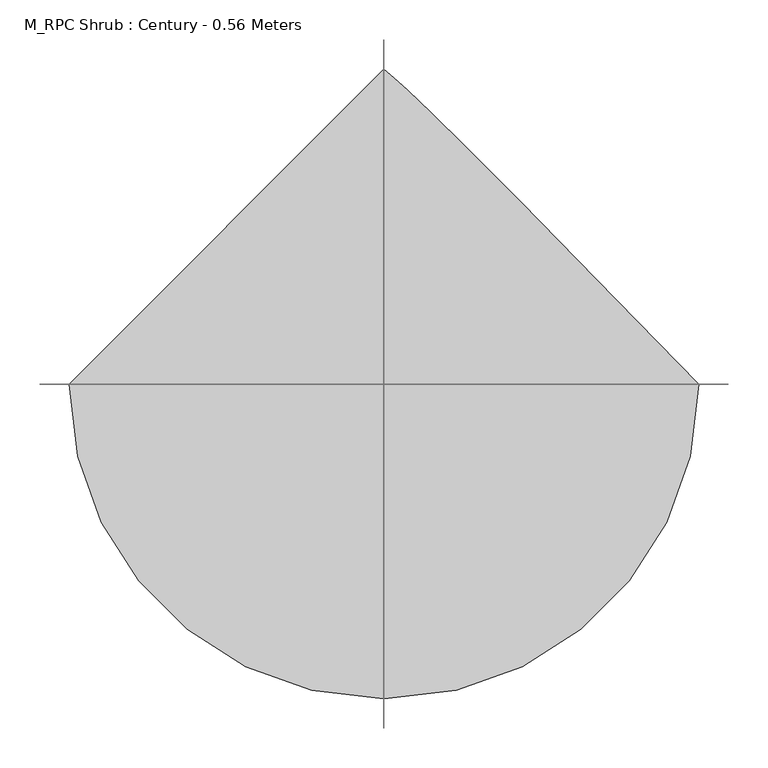
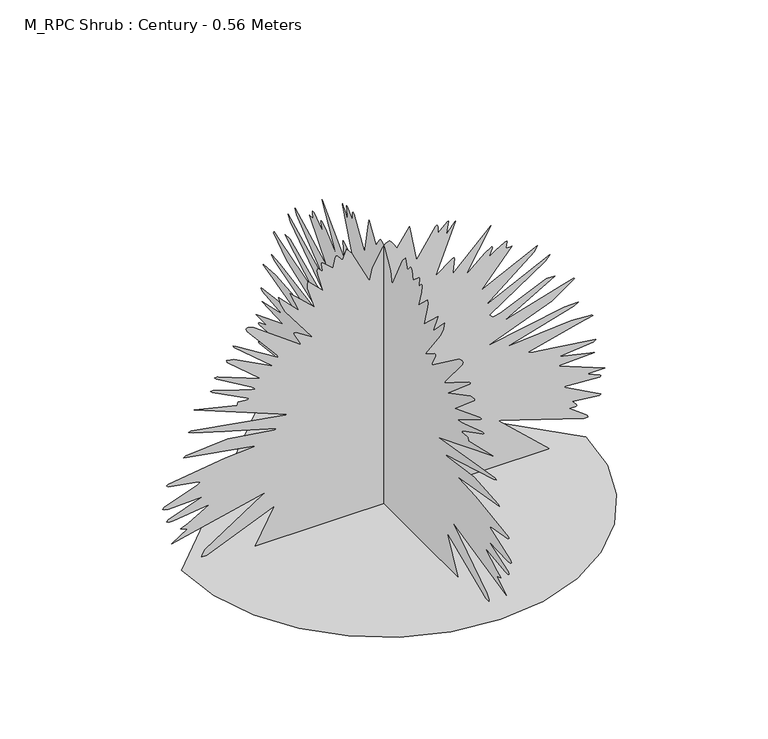
"""IFC4 building model written with IfcOpenShell, lengths in millimetres: geographic element geometry, M_RPC Shrub : Century - 0.56 Meters."""

from ifc_helpers import new_model, si_unit, origin, place, context, project, spatial, triangles, source, transform, mapped, element, save


def m_rpc_shrub_century_0_56_meters_67d26a43(model_context):
    return source(origin(), model_context, "Body", "Tessellation", [
        triangles([(-398.1646863, 0.0, 4.64e-05), (-387.6392386, -91.2330759, 4.64e-05), (-357.6589102, -175.0158616, 4.64e-05), (-310.62915, -248.9482674, 4.64e-05), (-248.9482674, -310.62915, 4.64e-05), (-175.0158616, -357.6589102, 4.64e-05), (-91.2330759, -387.6392386, 4.64e-05), (1.74e-05, -398.1646863, 4.64e-05), (91.2330759, -387.6392386, 4.64e-05), (175.0158616, -357.6589102, 4.64e-05), (248.9482674, -310.62915, 4.64e-05), (310.62915, -248.9482674, 4.64e-05), (357.6589102, -175.0158616, 4.64e-05), (387.6392386, -91.2330759, 4.64e-05), (398.1646863, 3.48e-05, 4.64e-05), (268.7691869, 132.7272546, 4.64e-05), (172.8430654, 230.4484337, 4.64e-05), (104.8064389, 298.9964298, 4.64e-05), (59.0817226, 344.2087501, 4.64e-05), (30.0910616, 371.9185412, 4.64e-05), (12.2565295, 387.9599676, 4.64e-05), (-5.22e-05, 398.1646863, 4.64e-05), (5.49e-05, 64.8497162, 484.8984183), (5.49e-05, 101.536553, 542.1176365), (5.49e-05, 104.7998259, 543.9987353), (5.48e-05, 106.0554996, 542.5580166), (5.48e-05, 106.6816787, 540.4605792), (5.49e-05, 106.3998917, 526.3994825), (5.49e-05, 126.0240573, 543.3318429), (5.49e-05, 127.1998031, 543.9987353), (5.49e-05, 124.5247847, 525.7834954), (5.49e-05, 123.9199888, 519.3689524), (5.49e-05, 123.9999166, 518.3991351), (5.49e-05, 126.4310728, 521.7234962), (5.49e-05, 129.404674, 525.5416497), (5.49e-05, 132.6114368, 529.4820342), (5.49e-05, 135.7433586, 533.1856599), (5.49e-05, 138.4909199, 536.2834723), (5.49e-05, 140.5461178, 538.4089239), (5.49e-05, 141.5999325, 539.2005544), (5.49e-05, 101.5999394, 438.4006751), (5.49e-05, 135.4317952, 463.1119211), (5.49e-05, 138.3997917, 464.0002753), (5.47e-05, 139.1298253, 461.7042672), (5.51e-05, 136.2157953, 434.8777433), (5.49e-05, 136.7999711, 431.9988493), (5.49e-05, 211.4496842, 505.8500464), (5.49e-05, 160.799778, 419.2003209), (5.45e-05, 199.0650477, 452.2453606), (5.47e-05, 210.839547, 460.3373812), (5.49e-05, 213.5998255, 460.8006523), (5.49e-05, 214.2417921, 458.8177428), (5.49e-05, 213.7067412, 456.0762677), (5.5e-05, 208.6102318, 443.5832076), (5.49e-05, 208.7998641, 441.6002981), (5.47e-05, 220.3880376, 450.0359387), (5.47e-05, 238.7186048, 461.4981025), (5.49e-05, 242.3998299, 462.3991739), (5.49e-05, 242.9542292, 460.7548339), (5.49e-05, 240.6740268, 448.6562991), (5.49e-05, 240.7997641, 447.9995441), (5.49e-05, 241.2714286, 448.0708334), (5.49e-05, 242.5398286, 447.9257478), (5.49e-05, 244.3852829, 447.6737283), (5.49e-05, 246.5886367, 447.426832), (5.49e-05, 248.9301908, 447.2919202), (5.49e-05, 251.1902999, 447.3810136), (5.49e-05, 253.1497915, 447.7984663), (5.49e-05, 192.7999141, 377.5999895), (5.49e-05, 303.1989713, 431.9988493), (5.49e-05, 297.1993375, 421.8501228), (5.49e-05, 199.199687, 342.3989405), (5.49e-05, 327.2000499, 404.8006911), (5.49e-05, 318.9502264, 393.7992551), (5.49e-05, 208.7998641, 319.9989633), (5.49e-05, 215.1998913, 313.5996809), (5.49e-05, 230.1625681, 316.3946048), (5.49e-05, 320.6811527, 356.7196507), (5.49e-05, 337.1502056, 356.6483614), (5.49e-05, 238.1998319, 298.4491704), (5.49e-05, 354.9760071, 333.6273102), (5.49e-05, 375.1996273, 339.1993175), (5.49e-05, 375.7138038, 337.4455001), (5.49e-05, 331.4993151, 306.2993271), (5.49e-05, 203.9999027, 257.5997561), (5.49e-05, 355.6938412, 284.8055446), (5.49e-05, 383.1999747, 286.3989974), (5.49e-05, 374.9501876, 280.4986309), (5.49e-05, 243.9996596, 241.5998061), (5.49e-05, 369.6149028, 252.730304), (5.48e-05, 410.4057632, 249.1238926), (5.49e-05, 411.9992343, 247.9998333), (5.49e-05, 387.0894539, 241.9686426), (5.49e-05, 285.2993553, 215.7497124), (5.49e-05, 290.8815363, 213.1882227), (5.49e-05, 337.9749372, 207.3566019), (5.49e-05, 416.616685, 196.3696635), (5.49e-05, 418.3985167, 195.1997676), (5.52e-05, 413.4781411, 191.71199), (5.49e-05, 346.4004041, 185.5998631), (5.49e-05, 415.1988573, 169.5999131), (5.49e-05, 343.2007447, 166.3997632), (5.49e-05, 436.0003129, 129.599911), (5.49e-05, 400.7992275, 129.599911), (5.49e-05, 426.360676, 118.4839198), (5.49e-05, 427.9999291, 116.7998474), (5.51e-05, 425.8286591, 115.4250494), (5.56e-05, 353.1509368, 119.8681376), (5.49e-05, 427.9999291, 78.3999202), (5.49e-05, 425.4595682, 76.8158872), (5.49e-05, 372.0000043, 83.1998816), (5.49e-05, 379.473458, 73.9621824), (5.49e-05, 380.2828926, 71.8871274), (5.49e-05, 380.0003517, 70.3998226), (5.5e-05, 378.39162, 69.8721477), (5.49e-05, 365.6007219, 70.3998226), (5.51e-05, 397.7981389, 47.0083907), (5.51e-05, 401.3999539, 43.1362478), (5.49e-05, 402.4003289, 39.9999976), (5.52e-05, 394.3261488, 39.8897799), (5.49e-05, 224.7995597, 94.3998702), (5.49e-05, 327.2000499, 0.0), (5.26e-05, -253.5998185, 0.2497534), (5.49e-05, -215.1998913, 70.3998226), (5.53e-05, -349.5058468, 14.9203965), (5.49e-05, -359.1989325, 14.3999784), (5.49e-05, -358.4582073, 18.4088623), (5.49e-05, -352.929475, 27.5733556), (5.49e-05, -237.8852254, 102.3824044), (5.49e-05, -229.5997755, 105.5998588), (5.49e-05, -418.3985167, 62.3999748), (5.49e-05, -386.3996341, 83.1998816), (5.49e-05, -400.0025102, 87.4296561), (5.49e-05, -400.7992275, 87.999843), (5.49e-05, -386.0559777, 93.9304857), (5.49e-05, -343.2007447, 118.3999223), (5.53e-05, -414.9570479, 109.1403313), (5.52e-05, -423.9373864, 109.6170918), (5.49e-05, -427.9999291, 111.999886), (5.47e-05, -424.9504786, 115.4097796), (5.49e-05, -357.6003745, 139.1998246), (5.52e-05, -424.695952, 136.9435397), (5.52e-05, -432.7879363, 138.2035373), (5.49e-05, -436.0003129, 140.7998996), (5.49e-05, -432.057385, 144.8611706), (5.51e-05, -366.8785509, 167.9405303), (5.49e-05, -362.3985555, 171.1997246), (5.48e-05, -365.5549035, 173.2315046), (5.52e-05, -424.548323, 183.6813392), (5.49e-05, -427.9999291, 187.1996746), (5.5e-05, -424.9912102, 188.5632723), (5.5e-05, -312.2404252, 204.2493606), (5.5e-05, -256.8437521, 207.9244815), (5.49e-05, -253.5998185, 209.5996518), (5.49e-05, -394.3999815, 233.5996948), (5.47e-05, -390.436706, 236.3123926), (5.49e-05, -308.2873235, 242.4260456), (5.52e-05, -215.1914979, 228.4782414), (5.49e-05, -210.3996938, 230.3998175), (5.5e-05, -317.0436931, 261.3695659), (5.51e-05, -375.8232811, 278.6964516), (5.49e-05, -384.7985327, 283.1993563), (5.48e-05, -379.7305281, 284.1615432), (5.49e-05, -186.3998869, 251.1997107), (5.49e-05, -373.5985259, 326.4007891), (5.49e-05, -288.7993597, 305.5993335), (5.49e-05, -287.2008017, 311.9986158), (5.5e-05, -269.6142843, 310.6546208), (5.5e-05, -267.4048262, 311.0720736), (5.49e-05, -266.3993824, 311.9986158), (5.52e-05, -270.0673635, 315.259318), (5.51e-05, -338.1327765, 350.2134707), (5.49e-05, -341.5996797, 353.5989109), (5.49e-05, -336.2949526, 353.3087397), (5.54e-05, -272.2895571, 332.4284008), (5.53e-05, -259.5164814, 328.6509424), (5.49e-05, -253.5998185, 327.9993107), (5.48e-05, -256.7444849, 331.695306), (5.51e-05, -330.0891177, 375.2072577), (5.49e-05, -333.5992959, 379.1985475), (5.48e-05, -328.2309463, 379.1425552), (5.49e-05, -242.3998299, 345.5985635), (5.51e-05, -308.8677023, 402.8279554), (5.49e-05, -309.6007971, 406.3992491), (5.49e-05, -295.3818975, 403.9785029), (5.49e-05, -218.3997869, 363.2003597), (5.5e-05, -295.1171608, 428.5930252), (5.49e-05, -296.7997071, 431.9988493), (5.43e-05, -290.6473573, 429.7792173), (5.43e-05, -242.0870038, 399.1116125), (5.49e-05, -207.1997983, 377.5999895), (5.5e-05, -209.9585506, 383.227989), (5.51e-05, -269.0008225, 453.4340961), (5.49e-05, -271.2001069, 459.1995509), (5.48e-05, -269.5073686, 460.136267), (5.48e-05, -267.1197418, 460.2660919), (5.49e-05, -256.5637546, 456.7737179), (5.49e-05, -163.9999097, 388.7999963), (5.51e-05, -163.8922309, 391.6330719), (5.51e-05, -177.0634292, 415.4890649), (5.49e-05, -176.7997098, 417.5992195), (5.46e-05, -172.6549592, 417.5126696), (5.49e-05, -139.9998666, 396.8003437), (5.49e-05, -194.1836233, 468.5159154), (5.49e-05, -203.5692241, 486.9984355), (5.49e-05, -207.1997983, 502.3984039), (5.49e-05, -167.1998052, 460.8006523), (5.49e-05, -184.799821, 502.3984039), (5.49e-05, -136.7999711, 457.5984495), (5.49e-05, -150.0974153, 501.1027708), (5.49e-05, -150.4718564, 508.5049716), (5.49e-05, -149.5997803, 515.1995121), (5.49e-05, -119.1999553, 486.4002525), (5.44e-05, -128.5677247, 518.5645683), (5.46e-05, -131.0228165, 531.0958529), (5.49e-05, -130.3999439, 534.39983), (5.48e-05, -129.2058761, 534.7740077), (5.48e-05, -127.886816, 534.1198325), (5.5e-05, -121.9235899, 527.8402013), (5.5e-05, -120.4008994, 527.0129262), (5.5e-05, -120.2359567, 529.3420355), (5.49e-05, -122.5647935, 541.6518219), (5.49e-05, -122.3998417, 543.9987353), (5.47e-05, -119.8953707, 543.5074499), (5.49e-05, -102.2846633, 527.55003), (5.49e-05, -99.9998645, 526.3994825), (5.47e-05, -96.0065581, 544.5052814), (5.48e-05, -94.9280538, 547.1169316), (5.49e-05, -93.5998373, 548.7994597), (5.48e-05, -91.4494416, 548.2191173), (5.49e-05, -80.8000281, 535.9983879), (5.49e-05, -73.8677477, 555.4583556), (5.49e-05, -73.4500361, 555.949641), (5.49e-05, -63.3254997, 544.6173022), (5.49e-05, -27.9999715, 473.5991807), (5.45e-05, -22.4632319, 499.4533439), (5.39e-05, -2.4030595, 534.758747), (5.42e-05, 4.5359445, 541.494019), (5.49e-05, 10.3999784, 543.9987353), (5.49e-05, 12.3719147, 542.8354706), (5.49e-05, 15.0237162, 539.8598528), (5.49e-05, 18.0101936, 535.7973101), (5.49e-05, 20.9862349, 531.3758503), (5.49e-05, 23.6065737, 527.315851), (5.49e-05, 25.5263012, 524.350407), (5.49e-05, 26.3999011, 523.1998595), (5.49e-05, 50.3999487, 559.9994665), (64.8497162, 5.25e-05, 484.8984183), (101.536553, 4.91e-05, 542.1176365), (104.7998259, 4.9e-05, 543.9987353), (106.0554996, 4.92e-05, 542.5580166), (106.6816787, 4.93e-05, 540.4605792), (106.3998917, 5e-05, 526.3994825), (126.0240573, 4.9e-05, 543.3318429), (127.1998031, 4.9e-05, 543.9987353), (124.5247847, 5e-05, 525.7834954), (123.9199888, 5.04e-05, 519.3689524), (123.9999166, 5.05e-05, 518.3991351), (126.4310728, 5.03e-05, 521.7234962), (129.404674, 5.01e-05, 525.5416497), (132.6114368, 4.98e-05, 529.4820342), (135.7433586, 4.96e-05, 533.1856599), (138.4909199, 4.94e-05, 536.2834723), (140.5461178, 4.93e-05, 538.4089239), (141.5999325, 4.92e-05, 539.2005544), (101.5999394, 5.52e-05, 438.4006751), (135.4317952, 5.38e-05, 463.1119211), (138.3997917, 5.37e-05, 464.0002753), (139.1298253, 5.41e-05, 461.7042672), (136.2157953, 5.53e-05, 434.8777433), (136.7999711, 5.56e-05, 431.9988493), (211.4496842, 5.12e-05, 505.8500464), (160.799778, 5.64e-05, 419.2003209), (199.0650477, 5.48e-05, 452.2453606), (210.839547, 5.42e-05, 460.3373812), (213.5998255, 5.39e-05, 460.8006523), (214.2417921, 5.41e-05, 458.8177428), (213.7067412, 5.43e-05, 456.0762677), (208.6102318, 5.49e-05, 443.5832076), (208.7998641, 5.51e-05, 441.6002981), (220.3880376, 5.48e-05, 450.0359387), (238.7186048, 5.41e-05, 461.4981025), (242.3998299, 5.38e-05, 462.3991739), (242.9542292, 5.4e-05, 460.7548339), (240.6740268, 5.46e-05, 448.6562991), (240.7997641, 5.47e-05, 447.9995441), (241.2714286, 5.47e-05, 448.0708334), (242.5398286, 5.47e-05, 447.9257478), (244.3852829, 5.47e-05, 447.6737283), (246.5886367, 5.47e-05, 447.426832), (248.9301908, 5.47e-05, 447.2919202), (251.1902999, 5.47e-05, 447.3810136), (253.1497915, 5.47e-05, 447.7984663), (192.7999141, 5.89e-05, 377.5999895), (303.1989713, 5.56e-05, 431.9988493), (297.1993375, 5.62e-05, 421.8501228), (199.199687, 6.1e-05, 342.3989405), (327.2000499, 5.73e-05, 404.8006911), (318.9502264, 5.79e-05, 393.7992551), (208.7998641, 6.23e-05, 319.9989633), (215.1998913, 6.27e-05, 313.5996809), (230.1625681, 6.25e-05, 316.3946048), (320.6811527, 6.01e-05, 356.7196507), (337.1502056, 6.01e-05, 356.6483614), (238.1998319, 6.36e-05, 298.4491704), (354.9760071, 6.15e-05, 333.6273102), (375.1996273, 6.12e-05, 339.1993175), (375.7138038, 6.13e-05, 337.4455001), (331.4993151, 6.31e-05, 306.2993271), (203.9999027, 6.6e-05, 257.5997561), (355.6938412, 6.44e-05, 284.8055446), (383.1999747, 6.43e-05, 286.3989974), (374.9501876, 6.47e-05, 280.4986309), (243.9996596, 6.7e-05, 241.5998061), (369.6149028, 6.63e-05, 252.730304), (410.4057632, 6.66e-05, 249.1238926), (411.9992343, 6.66e-05, 247.9998333), (387.0894539, 6.7e-05, 241.9686426), (285.2993553, 6.85e-05, 215.7497124), (290.8815363, 6.87e-05, 213.1882227), (337.9749372, 6.9e-05, 207.3566019), (416.616685, 6.97e-05, 196.3696635), (418.3985167, 6.97e-05, 195.1997676), (413.4781411, 6.96e-05, 191.71199), (346.4004041, 7.03e-05, 185.5998631), (415.1988573, 7.13e-05, 169.5999131), (343.2007447, 7.15e-05, 166.3997632), (436.0003129, 7.37e-05, 129.599911), (400.7992275, 7.37e-05, 129.599911), (426.360676, 7.43e-05, 118.4839198), (427.9999291, 7.44e-05, 116.7998474), (425.8286591, 7.43e-05, 115.4250494), (353.1509368, 7.36e-05, 119.8681376), (427.9999291, 7.67e-05, 78.3999202), (425.4595682, 7.68e-05, 76.8158872), (372.0000043, 7.64e-05, 83.1998816), (379.473458, 7.7e-05, 73.9621824), (380.2828926, 7.71e-05, 71.8871274), (380.0003517, 7.72e-05, 70.3998226), (378.39162, 7.71e-05, 69.8721477), (365.6007219, 7.72e-05, 70.3998226), (397.7981389, 7.84e-05, 47.0083907), (401.3999539, 7.87e-05, 43.1362478), (402.4003289, 7.9e-05, 39.9999976), (394.3261488, 7.87e-05, 39.8897799), (224.7995597, 7.58e-05, 94.3998702), (327.2000499, 8.14e-05, 1.09e-05), (-253.5998185, 8.37e-05, 0.2497643), (-215.1998913, 7.72e-05, 70.3998226), (-349.5058468, 8.01e-05, 14.9204215), (-359.1989325, 8.05e-05, 14.4000045), (-358.4582073, 8.03e-05, 18.4088623), (-352.929475, 7.97e-05, 27.5733556), (-237.8852254, 7.53e-05, 102.3824044), (-229.5997755, 7.51e-05, 105.5998588), (-418.3985167, 7.77e-05, 62.3999748), (-386.3996341, 7.64e-05, 83.1998816), (-400.0025102, 7.62e-05, 87.4296561), (-400.7992275, 7.61e-05, 87.999843), (-386.0559777, 7.58e-05, 93.9304857), (-343.2007447, 7.43e-05, 118.3999223), (-414.9570479, 7.46e-05, 109.1403313), (-423.9373864, 7.46e-05, 109.6170918), (-427.9999291, 7.47e-05, 111.999886), (-424.9504786, 7.47e-05, 115.4097796), (-357.6003745, 7.31e-05, 139.1998246), (-424.695952, 7.29e-05, 136.9435397), (-432.7879363, 7.29e-05, 138.2035373), (-436.0003129, 7.3e-05, 140.7998996), (-432.057385, 7.28e-05, 144.8611706), (-366.8785509, 7.12e-05, 167.9405303), (-362.3985555, 7.12e-05, 171.1997246), (-365.5549035, 7.11e-05, 173.2315046), (-424.548323, 7.02e-05, 183.6813392), (-427.9999291, 7.02e-05, 187.1996746), (-424.9912102, 7.01e-05, 188.5632723), (-312.2404252, 6.92e-05, 204.2493606), (-256.8437521, 6.89e-05, 207.9244815), (-253.5998185, 6.89e-05, 209.5996518), (-394.3999815, 6.75e-05, 233.5996948), (-390.436706, 6.75e-05, 236.3123926), (-308.2873235, 6.7e-05, 242.4260456), (-215.1914979, 6.75e-05, 228.4782414), (-210.3996938, 6.76e-05, 230.3998175), (-317.0436931, 6.57e-05, 261.3695659), (-375.8232811, 6.46e-05, 278.6964516), (-384.7985327, 6.45e-05, 283.1993563), (-379.7305281, 6.46e-05, 284.1615432), (-186.3998869, 6.64e-05, 251.1997107), (-373.5985259, 6.19e-05, 326.4007891), (-288.7993597, 6.32e-05, 305.5993335), (-287.2008017, 6.28e-05, 311.9986158), (-269.6142843, 6.28e-05, 310.6546208), (-267.4048262, 6.28e-05, 311.0720736), (-266.3993824, 6.28e-05, 311.9986158), (-270.0673635, 6.23e-05, 315.259318), (-338.1327765, 6.04e-05, 350.2134707), (-341.5996797, 6.03e-05, 353.5989109), (-336.2949526, 6.04e-05, 353.3087397), (-272.2895571, 6.11e-05, 332.4284008), (-259.5164814, 6.14e-05, 328.6509424), (-253.5998185, 6.18e-05, 327.9993107), (-256.7444849, 6.17e-05, 331.695306), (-330.0891177, 5.89e-05, 375.2072577), (-333.5992959, 5.88e-05, 379.1985475), (-328.2309463, 5.89e-05, 379.1425552), (-242.3998299, 6.08e-05, 345.5985635), (-308.8677023, 5.72e-05, 402.8279554), (-309.6007971, 5.72e-05, 406.3992491), (-295.3818975, 5.73e-05, 403.9785029), (-218.3997869, 5.97e-05, 363.2003597), (-295.1171608, 5.58e-05, 428.5930252), (-296.7997071, 5.56e-05, 431.9988493), (-290.6473573, 5.64e-05, 429.7792173), (-242.0870038, 5.82e-05, 399.1116125), (-207.1997983, 5.89e-05, 377.5999895), (-209.9585506, 5.85e-05, 383.227989), (-269.0008225, 5.42e-05, 453.4340961), (-271.2001069, 5.4e-05, 459.1995509), (-269.5073686, 5.41e-05, 460.136267), (-267.1197418, 5.41e-05, 460.2660919), (-256.5637546, 5.42e-05, 456.7737179), (-163.9999097, 5.82e-05, 388.7999963), (-163.8922309, 5.78e-05, 391.6330719), (-177.0634292, 5.65e-05, 415.4890649), (-176.7997098, 5.65e-05, 417.5992195), (-172.6549592, 5.68e-05, 417.5126696), (-139.9998666, 5.77e-05, 396.8003437), (-194.1836233, 5.35e-05, 468.5159154), (-203.5692241, 5.24e-05, 486.9984355), (-207.1997983, 5.14e-05, 502.3984039), (-167.1998052, 5.39e-05, 460.8006523), (-184.799821, 5.14e-05, 502.3984039), (-136.7999711, 5.41e-05, 457.5984495), (-150.0974153, 5.15e-05, 501.1027708), (-150.4718564, 5.11e-05, 508.5049716), (-149.5997803, 5.07e-05, 515.1995121), (-119.1999553, 5.24e-05, 486.4002525), (-128.5677247, 5.1e-05, 518.5645683), (-131.0228165, 5.01e-05, 531.0958529), (-130.3999439, 4.95e-05, 534.39983), (-129.2058761, 4.96e-05, 534.7740077), (-127.886816, 4.96e-05, 534.1198325), (-121.9235899, 4.98e-05, 527.8402013), (-120.4008994, 4.99e-05, 527.0129262), (-120.2359567, 4.97e-05, 529.3420355), (-122.5647935, 4.91e-05, 541.6518219), (-122.3998417, 4.9e-05, 543.9987353), (-119.8953707, 4.92e-05, 543.5074499), (-102.2846633, 5e-05, 527.55003), (-99.9998645, 5e-05, 526.3994825), (-96.0065581, 4.91e-05, 544.5052814), (-94.9280538, 4.89e-05, 547.1169316), (-93.5998373, 4.87e-05, 548.7994597), (-91.4494416, 4.88e-05, 548.2191173), (-80.8000281, 4.94e-05, 535.9983879), (-73.8677477, 4.83e-05, 555.4583556), (-73.4500361, 4.82e-05, 555.949641), (-63.3254997, 4.89e-05, 544.6173022), (-27.9999715, 5.32e-05, 473.5991807), (-22.4632319, 5.2e-05, 499.4533439), (-2.4030595, 5.05e-05, 534.758747), (4.5359445, 4.98e-05, 541.494019), (10.3999784, 4.9e-05, 543.9987353), (12.3719147, 4.9e-05, 542.8354706), (15.0237162, 4.92e-05, 539.8598528), (18.0101936, 4.94e-05, 535.7973101), (20.9862349, 4.97e-05, 531.3758503), (23.6065737, 4.99e-05, 527.315851), (25.5263012, 5.01e-05, 524.350407), (26.3999011, 5.02e-05, 523.1998595), (50.3999487, 4.8e-05, 559.9994665)], [[21, 22, 1], [20, 21, 1], [19, 20, 1], [18, 19, 1], [17, 18, 1], [17, 1, 2], [17, 2, 3], [17, 3, 4], [16, 17, 4], [16, 4, 5], [16, 5, 6], [16, 6, 7], [16, 7, 8], [16, 8, 9], [16, 9, 10], [16, 10, 11], [16, 11, 12], [15, 16, 12], [14, 15, 12], [13, 14, 12], [164, 165, 166], [46, 47, 48], [100, 101, 102], [130, 131, 132], [102, 103, 104], [207, 208, 209], [72, 73, 74], [72, 74, 75], [205, 206, 207], [204, 205, 207], [78, 79, 80], [39, 40, 41], [38, 39, 41], [37, 38, 41], [36, 37, 41], [35, 36, 41], [34, 35, 41], [33, 34, 41], [86, 87, 88], [86, 88, 89], [69, 70, 71], [69, 71, 72], [67, 68, 69], [161, 162, 163], [172, 173, 174], [121, 122, 123], [187, 188, 189], [246, 247, 23], [154, 155, 156], [154, 156, 157], [77, 78, 80], [66, 67, 69], [179, 180, 181], [91, 92, 93], [90, 91, 93], [121, 123, 124], [29, 30, 31], [133, 134, 135], [132, 133, 135], [211, 212, 213], [210, 211, 213], [65, 66, 69], [85, 86, 89], [64, 65, 69], [187, 189, 190], [186, 187, 190], [108, 109, 110], [108, 110, 111], [63, 64, 69], [62, 63, 69], [61, 62, 69], [97, 98, 99], [183, 184, 185], [149, 150, 151], [118, 119, 120], [117, 118, 120], [125, 126, 127], [105, 106, 107], [138, 139, 140], [160, 161, 163], [160, 163, 164], [159, 160, 164], [232, 233, 234], [231, 232, 234], [222, 223, 224], [186, 190, 191], [143, 144, 145], [96, 97, 99], [172, 174, 175], [171, 172, 175], [171, 175, 176], [81, 82, 83], [81, 83, 84], [42, 43, 44], [96, 99, 100], [182, 183, 185], [142, 143, 145], [141, 142, 145], [170, 171, 176], [203, 204, 207], [203, 207, 209], [141, 145, 146], [57, 58, 59], [89, 90, 93], [89, 93, 94], [81, 84, 85], [80, 81, 85], [200, 201, 202], [148, 149, 151], [148, 151, 152], [178, 179, 181], [178, 181, 182], [177, 178, 182], [193, 194, 195], [193, 195, 196], [166, 167, 168], [164, 166, 168], [164, 168, 169], [164, 169, 170], [50, 51, 52], [116, 117, 120], [24, 25, 26], [24, 26, 27], [137, 138, 140], [136, 137, 140], [136, 140, 141], [50, 52, 53], [49, 50, 53], [49, 53, 54], [49, 54, 55], [76, 77, 80], [76, 80, 85], [125, 127, 128], [124, 125, 128], [124, 128, 129], [124, 129, 130], [199, 200, 202], [182, 185, 186], [147, 148, 152], [164, 170, 176], [164, 176, 177], [104, 105, 107], [104, 107, 108], [102, 104, 108], [193, 196, 197], [192, 193, 197], [192, 197, 198], [191, 192, 198], [164, 177, 182], [164, 182, 186], [141, 146, 147], [130, 132, 135], [130, 135, 136], [121, 124, 130], [221, 222, 224], [28, 29, 31], [28, 31, 32], [41, 42, 44], [41, 44, 45], [23, 24, 27], [23, 27, 28], [209, 210, 213], [199, 202, 203], [198, 199, 203], [221, 224, 225], [220, 221, 225], [154, 157, 158], [228, 229, 230], [56, 57, 59], [56, 59, 60], [116, 120, 121], [28, 32, 33], [28, 33, 41], [23, 28, 41], [215, 216, 217], [215, 217, 218], [214, 215, 218], [214, 218, 219], [214, 219, 220], [113, 114, 115], [112, 113, 115], [111, 112, 115], [41, 45, 46], [111, 115, 116], [214, 220, 225], [214, 225, 226], [96, 100, 102], [56, 60, 61], [56, 61, 69], [55, 56, 69], [49, 55, 69], [48, 49, 69], [111, 116, 121], [108, 111, 121], [102, 108, 121], [96, 102, 121], [95, 96, 121], [94, 95, 121], [89, 94, 121], [89, 121, 130], [85, 89, 130], [76, 85, 130], [75, 76, 130], [72, 75, 130], [69, 72, 130], [48, 69, 130], [46, 48, 130], [41, 46, 130], [23, 41, 130], [246, 23, 130], [245, 246, 130], [244, 245, 130], [243, 244, 130], [242, 243, 130], [241, 242, 130], [240, 241, 130], [227, 228, 230], [227, 230, 231], [226, 227, 231], [141, 147, 152], [136, 141, 152], [130, 136, 152], [130, 152, 153], [130, 153, 154], [130, 154, 158], [130, 158, 159], [164, 186, 191], [164, 191, 198], [164, 198, 203], [238, 239, 240], [231, 234, 235], [226, 231, 235], [214, 226, 235], [213, 214, 235], [209, 213, 235], [203, 209, 235], [130, 159, 164], [164, 203, 235], [237, 238, 240], [236, 237, 240], [235, 236, 240], [235, 240, 130], [164, 235, 130], [389, 390, 391], [271, 272, 273], [325, 326, 327], [355, 356, 357], [327, 328, 329], [432, 433, 434], [297, 298, 299], [297, 299, 300], [430, 431, 432], [429, 430, 432], [303, 304, 305], [264, 265, 266], [263, 264, 266], [262, 263, 266], [261, 262, 266], [260, 261, 266], [259, 260, 266], [258, 259, 266], [311, 312, 313], [311, 313, 314], [294, 295, 296], [294, 296, 297], [292, 293, 294], [386, 387, 388], [397, 398, 399], [346, 347, 348], [412, 413, 414], [471, 472, 248], [379, 380, 381], [379, 381, 382], [302, 303, 305], [291, 292, 294], [404, 405, 406], [316, 317, 318], [315, 316, 318], [346, 348, 349], [254, 255, 256], [358, 359, 360], [357, 358, 360], [436, 437, 438], [435, 436, 438], [290, 291, 294], [310, 311, 314], [289, 290, 294], [412, 414, 415], [411, 412, 415], [333, 334, 335], [333, 335, 336], [288, 289, 294], [287, 288, 294], [286, 287, 294], [322, 323, 324], [408, 409, 410], [374, 375, 376], [343, 344, 345], [342, 343, 345], [350, 351, 352], [330, 331, 332], [363, 364, 365], [385, 386, 388], [385, 388, 389], [384, 385, 389], [457, 458, 459], [456, 457, 459], [447, 448, 449], [411, 415, 416], [368, 369, 370], [321, 322, 324], [397, 399, 400], [396, 397, 400], [396, 400, 401], [306, 307, 308], [306, 308, 309], [267, 268, 269], [321, 324, 325], [407, 408, 410], [367, 368, 370], [366, 367, 370], [395, 396, 401], [428, 429, 432], [428, 432, 434], [366, 370, 371], [282, 283, 284], [314, 315, 318], [314, 318, 319], [306, 309, 310], [305, 306, 310], [425, 426, 427], [373, 374, 376], [373, 376, 377], [403, 404, 406], [403, 406, 407], [402, 403, 407], [418, 419, 420], [418, 420, 421], [391, 392, 393], [389, 391, 393], [389, 393, 394], [389, 394, 395], [275, 276, 277], [341, 342, 345], [249, 250, 251], [249, 251, 252], [362, 363, 365], [361, 362, 365], [361, 365, 366], [275, 277, 278], [274, 275, 278], [274, 278, 279], [274, 279, 280], [301, 302, 305], [301, 305, 310], [350, 352, 353], [349, 350, 353], [349, 353, 354], [349, 354, 355], [424, 425, 427], [407, 410, 411], [372, 373, 377], [389, 395, 401], [389, 401, 402], [329, 330, 332], [329, 332, 333], [327, 329, 333], [418, 421, 422], [417, 418, 422], [417, 422, 423], [416, 417, 423], [389, 402, 407], [389, 407, 411], [366, 371, 372], [355, 357, 360], [355, 360, 361], [346, 349, 355], [446, 447, 449], [253, 254, 256], [253, 256, 257], [266, 267, 269], [266, 269, 270], [248, 249, 252], [248, 252, 253], [434, 435, 438], [424, 427, 428], [423, 424, 428], [446, 449, 450], [445, 446, 450], [379, 382, 383], [453, 454, 455], [281, 282, 284], [281, 284, 285], [341, 345, 346], [253, 257, 258], [253, 258, 266], [248, 253, 266], [440, 441, 442], [440, 442, 443], [439, 440, 443], [439, 443, 444], [439, 444, 445], [338, 339, 340], [337, 338, 340], [336, 337, 340], [266, 270, 271], [336, 340, 341], [439, 445, 450], [439, 450, 451], [321, 325, 327], [281, 285, 286], [281, 286, 294], [280, 281, 294], [274, 280, 294], [273, 274, 294], [336, 341, 346], [333, 336, 346], [327, 333, 346], [321, 327, 346], [320, 321, 346], [319, 320, 346], [314, 319, 346], [314, 346, 355], [310, 314, 355], [301, 310, 355], [300, 301, 355], [297, 300, 355], [294, 297, 355], [273, 294, 355], [271, 273, 355], [266, 271, 355], [248, 266, 355], [471, 248, 355], [470, 471, 355], [469, 470, 355], [468, 469, 355], [467, 468, 355], [466, 467, 355], [465, 466, 355], [452, 453, 455], [452, 455, 456], [451, 452, 456], [366, 372, 377], [361, 366, 377], [355, 361, 377], [355, 377, 378], [355, 378, 379], [355, 379, 383], [355, 383, 384], [389, 411, 416], [389, 416, 423], [389, 423, 428], [463, 464, 465], [456, 459, 460], [451, 456, 460], [439, 451, 460], [438, 439, 460], [434, 438, 460], [428, 434, 460], [355, 384, 389], [389, 428, 460], [462, 463, 465], [461, 462, 465], [460, 461, 465], [460, 465, 355], [389, 460, 355]], closed=False),
    ])


if __name__ == "__main__":
    model = new_model("IFC4")
    model_context = context("Model", 3, world=origin())
    ifc_project = project(units=[si_unit("LENGTHUNIT", "METRE", prefix="MILLI")], contexts=[model_context])
    site = spatial("IfcSite", under=ifc_project)
    building = spatial("IfcBuilding", under=site)
    placement = place(None, origin())
    m_rpc_shrub_century_0_56_meters_shape = m_rpc_shrub_century_0_56_meters_67d26a43(model_context)
    element("IfcGeographicElement", 1, ObjectType="M_RPC Shrub : Century - 0.56 Meters", at=placement, inside=building, context=model_context, shape_type="MappedRepresentation", body=[
        mapped(m_rpc_shrub_century_0_56_meters_shape, transform((0.0, 0.0, 0.0), x_axis=(1.0, 0.0, 0.0), y_axis=(0.0, 1.0, 0.0), z_axis=(0.0, 0.0, 1.0))),
    ])
    save(model, "model.ifc")

# Revit data of these elements
# Type "M_RPC Shrub : Century - 0.56 Meters"
#   Type Comments = "Century"
#   built-in parameter 1005198 = "{2, 15},{39, RPC-16-FXAD-JSXX-UCRP-S000-ST1L-LVER-AU},{1, 0},{1, 0},{2, 35},{1, 8},{5, Color},{1, 0},{1, 0},{3, 0.8},{3, 0.8},{3, 0.8},{1, 8},{7, BBoxMin},{1, 0},{1, 0},{1, 0},{1, 0},{1, 0},{1, 8},{7, BBoxMax},{1, 0},{1, 0},{1, 0},{1, 0},{1, 0},{2, 11},{9, RPCTypeId},{1, 0},{1, 0},{39, RPC-16-FXAD-JSXX-UCRP-S000-ST1L-LVER-AU},{1, 6},{14, RPCPlantHeight},{1, 0},{1, 0},{7, 1.83727},{2, 11},{7, keyword},{1, 0},{1, 0},{21, :Geometry:RPC:Century},{2, 11},{8, category},{1, 0},{1, 0},{17, :Shrubs & Grasses},{2, 11},{12, LocalizedUID},{1, 0},{1, 0},{7, Century},{2, 14},{6, Height},{1, 0},{1, 0},{7, 1.83727},{1, 2},{16, Cast Reflections},{1, 0},{1, 0},{1, 0},{1, 2},{12, Cast Shadows},{1, 0},{1, 0},{1, 1},{1, 2},{9, Lock View},{1, 0},{1, 0},{1, 0},{1, 4},{5, ViewC},{1, 0},{1, 0},{1, 0},{2, 11},{20, AdvancedUIDefinition},{1, 0},{1, 0},{0, },{2, 11},{10, AssetLibID},{1, 0},{1, 0},{36, 4D3F6E72-3F99-4203-98E9-AF80B3C7A7A4},{2, 11},{10, BaseSchema},{1, 0},{1, 0},{9, RPCSchema},{2, 11},{12, ExchangeGUID},{1, 0},{1, 0},{0, },{1, 2},{6, Hidden},{1, 0},{1, 0},{1, 0},{1, 4},{11, RPCCategory},{1, 0},{1, 0},{1, 0},{2, 11},{8, RPCImage},{1, 0},{1, 0},{0, },{1, 4},{13, SchemaVersion},{1, 0},{1, 0},{1, 4},{2, 11},{12, UIDefinition},{1, 0},{1, 0},{0, },{2, 11},{6, UIName},{1, 0},{1, 0},{39, RPC-16-FXAD-JSXX-UCRP-S000-ST1L-LVER-AU},{2, 11},{11, VersionGUID},{1, 0},{1, 0},{9, RPCSchema},{2, 11},{9, assettype},{1, 0},{1, 0},{11, RPCGeometry},{2, 11},{11, description},{1, 0},{1, 0},{0, },{2, 11},{9, localname},{1, 0},{1, 0},{3, RPC},{2, 11},{9, localtype},{1, 0},{1, 0},{3, RPC},{1, 4},{8, revision},{1, 0},{1, 0},{1, 1},{2, 11},{9, thumbnail},{1, 0},{1, 0},{0, },{1, 4},{7, version},{1, 0},{1, 0},{1, 1},{1, 2},{20, RPC_Cast Reflections},{1, 0},{1, 0},{1, 1},{1, 2},{16, RPC_Cast Shadows},{1, 0},{1, 0},{1, 1},{1, 2},{13, RPC_Lock View},{1, 0},{1, 0},{1, 0},{1, 4},{9, RPC_ViewC},{1, 0},{1, 0},{1, 0},{21, assetlibrary_base.fbx},{1, 5},"
#   built-in parameter 1005195 = "RPC-16-FXAD-JSXX-UCRP-S000-ST1L-LVER-AU"
#   Height = 0.56 m
#   Description = (empty or 0)
#   Default Elevation = 0
